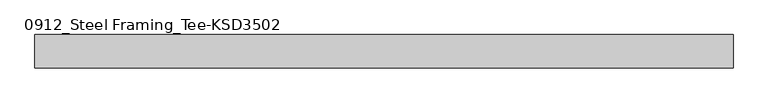
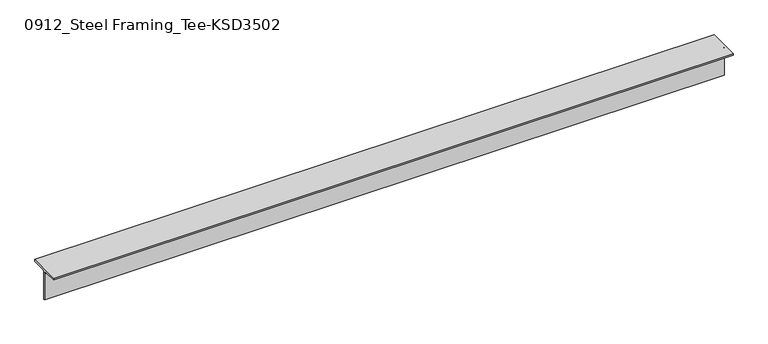
"""IFC4 building model written with IfcOpenShell, lengths in millimetres: member geometry, 0912_Steel Framing_Tee-KSD3502 : H_SB_ASB_CT-150x150x6.5x9."""

from ifc_helpers import new_model, si_unit, point, frame, frame_2d, origin, place, context, project, spatial, polyline, circle_curve, trimmed, segment, composite_curve, outline, extrude, source, transform, mapped, element, save


def member_0912_steel_framing_tee_ksd3502_fd058821(model_context):
    return source(origin(), model_context, "Body", "SweptSolid", [
        extrude(outline(composite_curve([segment(polyline([(-75.0, 75.0), (75.0, 75.0), (75.0, 66.0), (16.25, 66.0)]), True, "CONTINUOUS"), segment(trimmed(circle_curve(frame_2d((16.25, 53.0)), 13.0), [point((16.25, 66.0))], [point((3.25, 53.0))], True, "CARTESIAN"), True, "CONTINUOUS"), segment(polyline([(3.25, 53.0), (3.25, -75.0), (-3.25, -75.0), (-3.25, 53.0)]), True, "CONTINUOUS"), segment(trimmed(circle_curve(frame_2d((-16.25, 53.0)), 13.0), [point((-3.25, 53.0))], [point((-16.25, 66.0))], True, "CARTESIAN"), True, "CONTINUOUS"), segment(polyline([(-16.25, 66.0), (-75.0, 66.0), (-75.0, 75.0)]), True, "CONTINUOUS")], self_intersect=False)), frame((-1516.0, 0.0, 0.0), z_axis=(1.0, 0.0, 0.0), x_axis=(0.0, 1.0, 0.0)), (0.0, 0.0, 1.0), 3133.1),
    ])


if __name__ == "__main__":
    model = new_model("IFC4")
    model_context = context("Model", 3, world=origin())
    ifc_project = project(units=[si_unit("LENGTHUNIT", "METRE", prefix="MILLI")], contexts=[model_context])
    site = spatial("IfcSite", under=ifc_project)
    building = spatial("IfcBuilding", under=site)
    placement = place(None, origin())
    member_0912_steel_framing_tee_ksd3502_shape = member_0912_steel_framing_tee_ksd3502_fd058821(model_context)
    element("IfcMember", 1, ObjectType="0912_Steel Framing_Tee-KSD3502 : H_SB_ASB_CT-150x150x6.5x9", at=placement, inside=building, context=model_context, shape_type="MappedRepresentation", body=[
        mapped(member_0912_steel_framing_tee_ksd3502_shape, transform((0.0, 0.0, 0.0), x_axis=(1.0, 0.0, 0.0), y_axis=(0.0, 1.0, 0.0), z_axis=(0.0, 0.0, 1.0))),
    ])
    save(model, "model.ifc")

# Revit data of these elements
# Type "0912_Steel Framing_Tee-KSD3502 : H_SB_ASB_CT-150x150x6.5x9"
#   H_WM Code_1 = "S01AA003-00001 | Main Steel Structure Fabrication Work | Shelter/Building | Light Steel - Standard (30KG/M>Weight) | Material: (   )"
#   H_WM Code_2 = "S03AA029-00001 | Main Steel Structure Erection Work | Shelter/Building | Light Steel (30KG/M>Weight) | Material: (   )"
#   H_WM Code_3 = "S01AA010-00001 | Main Steel Structure Fabrication Work | Shelter/Building | Steel Painting/Coating | for Non-Fireproofed Steel Surface, Surface Preparation, Primer, Second & Final Coat | Material: (   )"
#   H_Q'ty Cal Type Tag = "SB-Q2"
#   Width = 15.0 cm
#   Web Thickness = 0.65 cm
#   Web Fillet = 1.3 cm
#   Section Area = 23.39 cm²
#   Perimeter = 0.60 m²/m
#   Nominal Weight = 18.40 kgf/m
#   Height = 15.0 cm
#   Flange Thickness = 0.9 cm
#   Centroid Vertical = 7.5 cm
#   Centroid Horizontal = 7.5 cm
#   Length [instance default] = 1.5000 m
#   Structural Material [instance default] = Steel, 45-345
#   Warping Constant = (empty or 0)
#   Torsional Moment of Inertia = 0
#   Section Name Key = ""
#   Plastic Modulus weak axis = 0
#   Plastic Modulus strong axis = 0
#   Moment of Inertia weak axis = 0
#   Moment of Inertia strong axis = 0
#   Elastic Modulus weak axis = 0
#   Elastic Modulus strong axis = 0
#   Bolt Spacing = 0
#   Assembly Code = ""
# Element 1 (IfcMember, "0912_Steel Framing_Tee-KSD3502 : H_SB_ASB_CT-150x150x6.5x9")
#   Structural Material = none
# Materials
#   "Steel, 45-345": class "Metal", colour RGB 189 187 185, transparency 0, Description = "Steel 345 MPa", Cost = 0
